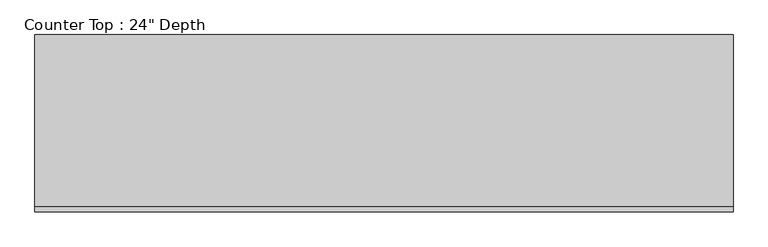
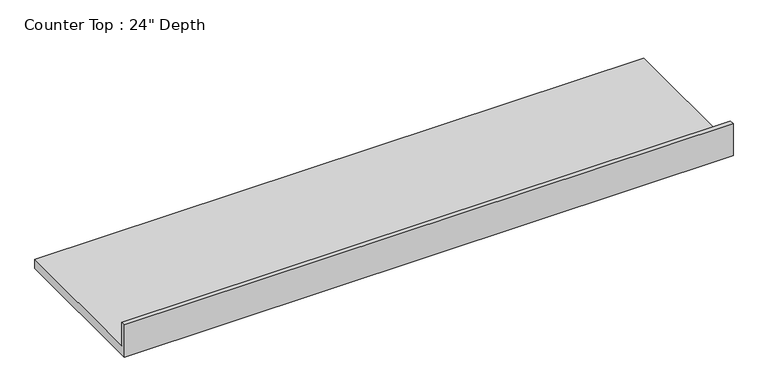
"""IFC4 building model written with IfcOpenShell, lengths in millimetres: furniture geometry."""

from ifc_helpers import new_model, si_unit, frame, origin, place, context, project, spatial, polyline, outline, extrude, source, transform, mapped, element, save


def furniture_58bfe37c(model_context):
    return source(origin(), model_context, "Body", "SweptSolid", [
        extrude(outline(polyline([(0.0, 1016.0), (19.05, 1016.0), (19.05, 914.4), (635.0, 914.4), (635.0, 876.3), (0.0, 876.3), (0.0, 1016.0)])), frame((-1200.4622951, 0.0, 0.0), z_axis=(1.0, 0.0, 0.0), x_axis=(0.0, 1.0, 0.0)), (0.0, 0.0, 1.0), 2497.1375),
    ])


if __name__ == "__main__":
    model = new_model("IFC4")
    model_context = context("Model", 3, world=origin())
    ifc_project = project(units=[si_unit("LENGTHUNIT", "METRE", prefix="MILLI")], contexts=[model_context])
    site = spatial("IfcSite", under=ifc_project)
    building = spatial("IfcBuilding", under=site)
    placement = place(None, origin())
    furniture_shape = furniture_58bfe37c(model_context)
    element("IfcFurniture", 1, ObjectType="Counter Top : 24\" Depth", at=placement, inside=building, context=model_context, shape_type="MappedRepresentation", body=[
        mapped(furniture_shape, transform((0.0, 0.0, 0.0), x_axis=(1.0, 0.0, 0.0), y_axis=(0.0, 1.0, 0.0), z_axis=(0.0, 0.0, 1.0))),
    ])
    save(model, "model.ifc")

# Revit data of these elements
# Type "Counter Top : 24\" Depth"
#   Assembly Code = "C1030400"
#   Counter Thickness = 0' - 1 1/2"
#   Depth = 2' - 1"
#   Height = 3' - 0"
#   Length [instance default] = 8' - 0"
#   Counter Top Material = none
# Element 1 (IfcFurniture, "Counter Top : 24\" Depth")
#   Length = 8' - 2 5/16"
#   Materials on its faces: "Counter Top"
# Materials
#   "Counter Top": class "Wood", colour RGB 226 177 128, transparency 0, Cost = 0
